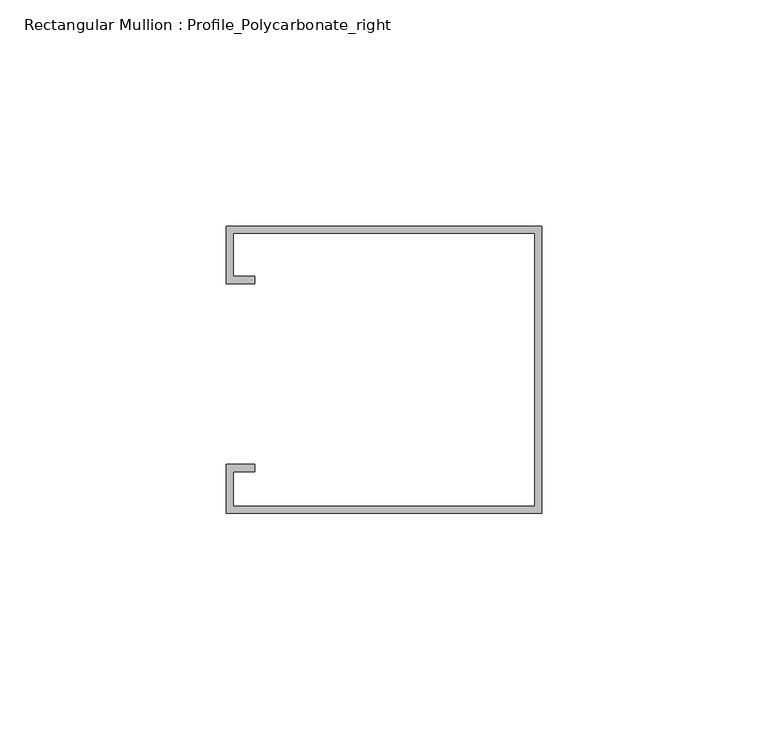
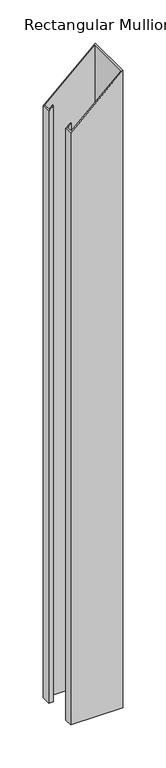
"""IFC4 building model written with IfcOpenShell, lengths in millimetres: member geometry, Rectangular Mullion : Profile_Polycarbonate_right."""

from ifc_helpers import new_model, si_unit, origin, place, context, project, spatial, faceted_brep, source, transform, mapped, element, save


def rectangular_mullion_profile_polycarbonate_right_72991202(model_context):
    return source(origin(), model_context, "Body", "Brep", [
        faceted_brep([(0.0, 32.7, -902.0076584), (0.0, -30.8, -902.0076584), (-69.85, -30.8, -902.0076584), (-69.85, -20.0, -902.0076584), (-63.5, -20.0, -902.0076584), (-63.5, -21.5875, -902.0076584), (-68.2625, -21.5875, -902.0076584), (-68.2625, -29.2125, -902.0076584), (-1.5875, -29.2125, -902.0076584), (-1.5875, 31.1125, -902.0076584), (-68.2625, 31.1125, -902.0076584), (-68.2625, 21.5875, -902.0076584), (-63.5, 21.5875, -902.0076584), (-63.5, 20.0, -902.0076584), (-69.85, 20.0, -902.0076584), (-69.85, 32.7, -902.0076584), (-69.85, 32.7, -64.2712818), (0.0, 32.7, 0.0), (-69.85, 20.0, -64.2712818), (-63.5, 20.0, -58.428438), (-63.5, 21.5875, -58.428438), (-68.2625, 21.5875, -62.8105708), (-68.2625, 31.1125, -62.8105708), (-1.5875, 31.1125, -1.4607109), (-1.5875, -29.2125, -1.4607109), (-68.2625, -29.2125, -62.8105708), (-68.2625, -21.5875, -62.8105708), (-63.5, -21.5875, -58.428438), (-63.5, -20.0, -58.428438), (-69.85, -20.0, -64.2712818), (-69.85, -30.8, -64.2712818), (0.0, -30.8, 0.0)], [[[0, 1, 2, 3, 4, 5, 6, 7, 8, 9, 10, 11, 12, 13, 14, 15]], [[16, 17, 0, 15]], [[18, 16, 15, 14]], [[19, 18, 14, 13]], [[20, 19, 13, 12]], [[21, 20, 12, 11]], [[22, 21, 11, 10]], [[23, 22, 10, 9]], [[24, 23, 9, 8]], [[25, 24, 8, 7]], [[26, 25, 7, 6]], [[27, 26, 6, 5]], [[28, 27, 5, 4]], [[29, 28, 4, 3]], [[30, 29, 3, 2]], [[31, 30, 2, 1]], [[17, 31, 1, 0]], [[17, 16, 18, 19, 20, 21, 22, 23, 24, 25, 26, 27, 28, 29, 30, 31]]]),
    ])


if __name__ == "__main__":
    model = new_model("IFC4")
    model_context = context("Model", 3, world=origin())
    ifc_project = project(units=[si_unit("LENGTHUNIT", "METRE", prefix="MILLI")], contexts=[model_context])
    site = spatial("IfcSite", under=ifc_project)
    building = spatial("IfcBuilding", under=site)
    placement = place(None, origin())
    rectangular_mullion_profile_polycarbonate_right_shape = rectangular_mullion_profile_polycarbonate_right_72991202(model_context)
    element("IfcMember", 1, ObjectType="Rectangular Mullion : Profile_Polycarbonate_right", at=placement, inside=building, context=model_context, shape_type="MappedRepresentation", body=[
        mapped(rectangular_mullion_profile_polycarbonate_right_shape, transform((0.0, 0.0, 0.0), x_axis=(1.0, 0.0, 0.0), y_axis=(0.0, 1.0, 0.0), z_axis=(0.0, 0.0, 1.0))),
    ])
    save(model, "model.ifc")

# Revit data of these elements
# Type "Rectangular Mullion : Profile_Polycarbonate_right"
#   built-in parameter 1007322 = 0.208333 (stored number, unit not read)
#   built-in parameter 1007321 = 0 (stored number, unit not read)
#   built-in parameter 1007320 = 0.00520833 (stored number, unit not read)
# Element 1 (IfcMember, "Rectangular Mullion : Profile_Polycarbonate_right")
#   Materials on its faces: "ALUMINUM PROFILE AT POLYCARBONATE PANEL"
# Materials
#   "ALUMINUM PROFILE AT POLYCARBONATE PANEL": class "Metal", colour RGB 244 244 244, transparency 0, Description = "Aluminum 6061", Cost = 0
